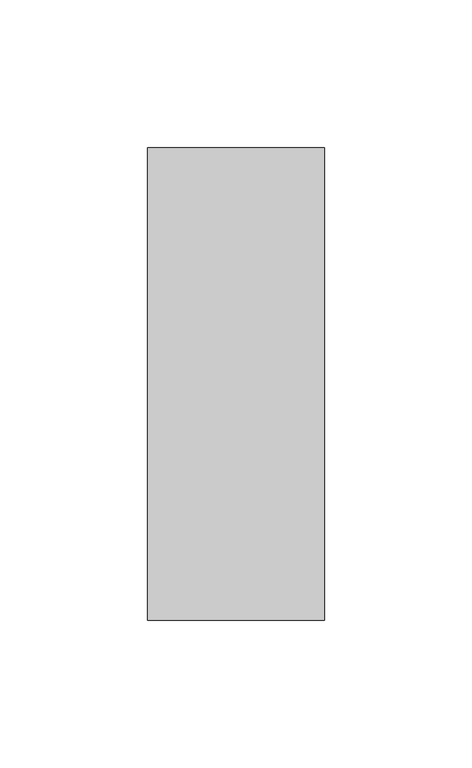
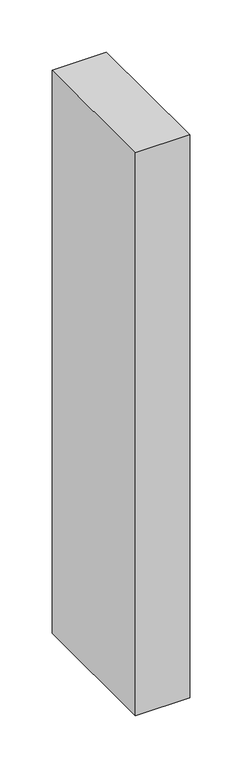
"""IFC4 building model written with IfcOpenShell, lengths in millimetres: column geometry, Madeira de lei-Coluna : Pontalete 6X16cm."""

import ifcopenshell
import ifcopenshell.guid

model = None  # the IFC model being written
_history = None  # IfcOwnerHistory: only IFC2X3 demands one
_inside = {}  # id of a spatial element -> (the spatial element, [elements in it])
_under = {}  # id of a project, library or spatial element -> (it, [spatial elements below it])
_declared = {}  # id of a project -> (the project, [libraries it declares])
_typed = {}  # id of a type object -> (the type object, [elements of that type])
_made_of = {}  # id of a material, layer set ... -> (it, [elements and type objects made of it])


def new_model(schema):
    """Start an empty IFC model of exactly this schema.

    Asked for "IFC4X3", IfcOpenShell would pick the latest addendum, in which some entities
    have other attributes; the version numbers below select the first issue.
    IFC2X3 requires an IfcOwnerHistory on every rooted entity: one is made here for all.
    """
    global model, _history
    if schema == "IFC4X3":
        model = ifcopenshell.file(schema_version=(4, 3, 0, 0))
    else:
        model = ifcopenshell.file(schema=schema)
    _inside.clear()
    _under.clear()
    _declared.clear()
    _typed.clear()
    _made_of.clear()
    _history = None
    if model.schema == "IFC2X3":
        org = make("IfcOrganization", Name="unknown")
        user = make(
            "IfcPersonAndOrganization",
            ThePerson=make("IfcPerson", FamilyName="unknown"),
            TheOrganization=org,
        )
        app = make(
            "IfcApplication",
            ApplicationDeveloper=org,
            Version="unknown",
            ApplicationFullName="unknown",
            ApplicationIdentifier="unknown",
        )
        _history = make(
            "IfcOwnerHistory",
            OwningUser=user,
            OwningApplication=app,
            ChangeAction="ADDED",
            CreationDate=0,
        )
    return model


def make(cls, **values):
    """One entity of the class cls with the attributes given. An attribute that is None is left unset."""
    return model.create_entity(
        cls, **{name: value for name, value in values.items() if value is not None}
    )


def rooted(cls, **values):
    """An entity with a GlobalId (a new one), such as an element, a storey or a relation."""
    return make(cls, GlobalId=ifcopenshell.guid.new(), OwnerHistory=_history, **values)


def si_unit(unit_type, name, prefix=None):
    """IfcSIUnit, for example si_unit("LENGTHUNIT", "METRE", prefix="MILLI")."""
    return make("IfcSIUnit", UnitType=unit_type, Prefix=prefix, Name=name)


def assignment(units):
    """IfcUnitAssignment: the units of a project."""
    return None if units is None else make("IfcUnitAssignment", Units=units)


def point(xyz):
    """IfcCartesianPoint."""
    return None if xyz is None else make("IfcCartesianPoint", Coordinates=xyz)


def direction(xyz):
    """IfcDirection."""
    return None if xyz is None else make("IfcDirection", DirectionRatios=xyz)


def frame(location, z_axis=None, x_axis=None):
    """IfcAxis2Placement3D, a coordinate frame: its origin and axes. An axis left out is left unset."""
    return make(
        "IfcAxis2Placement3D",
        Location=point(location),
        Axis=direction(z_axis),
        RefDirection=direction(x_axis),
    )


def origin():
    """The frame at (0, 0, 0) with its axes left unset."""
    return frame((0.0, 0.0, 0.0))


def place(relative_to, where):
    """IfcLocalPlacement: puts the frame where relative to a parent placement (None: the world)."""
    return make(
        "IfcLocalPlacement", PlacementRelTo=relative_to, RelativePlacement=where
    )


def context(
    kind, dimensions, precision=None, world=None, true_north=None, identifier=None
):
    """IfcGeometricRepresentationContext, for example the 3D "Model" context."""
    return make(
        "IfcGeometricRepresentationContext",
        ContextIdentifier=identifier,
        ContextType=kind,
        CoordinateSpaceDimension=dimensions,
        Precision=precision,
        WorldCoordinateSystem=world,
        TrueNorth=true_north,
    )


def project(units=None, contexts=None):
    """IfcProject with its units and contexts."""
    return rooted(
        "IfcProject",
        Name="project",
        RepresentationContexts=contexts,
        UnitsInContext=assignment(units),
    )


def spatial(cls, under=None, at=None, **own):
    """A site, building, storey or space (cls), placed at a placement, below another one or the project."""
    s = rooted(cls, ObjectPlacement=at, **own)
    if under is not None:
        _under.setdefault(under.id(), (under, []))[1].append(s)
    return s


def polyline(points):
    """IfcPolyline through the points."""
    return make("IfcPolyline", Points=[point(p) for p in points])


def outline(outer, holes=None, kind="AREA"):
    """IfcArbitraryClosedProfileDef: a profile drawn as a closed curve; with holes, ...WithVoids."""
    if holes is None:
        return make("IfcArbitraryClosedProfileDef", ProfileType=kind, OuterCurve=outer)
    return make(
        "IfcArbitraryProfileDefWithVoids",
        ProfileType=kind,
        OuterCurve=outer,
        InnerCurves=holes,
    )


def extrude(swept, where, along, depth):
    """IfcExtrudedAreaSolid: the profile swept, set in the frame where, extruded along a direction by depth."""
    return make(
        "IfcExtrudedAreaSolid",
        SweptArea=swept,
        Position=where,
        ExtrudedDirection=direction(along),
        Depth=depth,
    )


def shape(context_of_items, identifier, shape_type, items):
    """IfcShapeRepresentation: the items that make up one representation, for example the "Body"."""
    return make(
        "IfcShapeRepresentation",
        ContextOfItems=context_of_items,
        RepresentationIdentifier=identifier,
        RepresentationType=shape_type,
        Items=items,
    )


def source(mapping_origin, context_of_items, identifier, shape_type, items):
    """IfcRepresentationMap: a shape defined once, which mapped items show again and again."""
    return make(
        "IfcRepresentationMap",
        MappingOrigin=mapping_origin,
        MappedRepresentation=shape(context_of_items, identifier, shape_type, items),
    )


def transform(
    local_origin,
    x_axis=None,
    y_axis=None,
    z_axis=None,
    scale=None,
    scale2=None,
    scale3=None,
    uniform=True,
):
    """IfcCartesianTransformationOperator3D, or its non-uniform kind. x_axis, y_axis, z_axis: its Axis1, 2, 3."""
    if uniform:
        return make(
            "IfcCartesianTransformationOperator3D",
            Axis1=direction(x_axis),
            Axis2=direction(y_axis),
            LocalOrigin=point(local_origin),
            Scale=scale,
            Axis3=direction(z_axis),
        )
    return make(
        "IfcCartesianTransformationOperator3DnonUniform",
        Axis1=direction(x_axis),
        Axis2=direction(y_axis),
        LocalOrigin=point(local_origin),
        Scale=scale,
        Axis3=direction(z_axis),
        Scale2=scale2,
        Scale3=scale3,
    )


def mapped(mapping_source, mapping_target):
    """IfcMappedItem: shows the shape of a source again, moved by a transform."""
    return make(
        "IfcMappedItem", MappingSource=mapping_source, MappingTarget=mapping_target
    )


def made_of(thing, what):
    """Note that an element or type object is made of a material, layer set ...; save() writes the relation."""
    if what is not None:
        _made_of.setdefault(what.id(), (what, []))[1].append(thing)
    return thing


def element(
    cls,
    number,
    at=None,
    inside=None,
    cuts=None,
    type_object=None,
    material=None,
    context=None,
    identifier="Body",
    shape_type=None,
    held_by="IfcProductDefinitionShape",
    body=None,
    shapes=None,
    **own,
):
    """One element of the class cls, such as IfcWall. Its Tag is "e" and its number.

    at: its placement. inside: the storey or other place that contains it. cuts: it is an
    opening in that element (IfcRelVoidsElement). A single representation is given by context,
    identifier, shape_type and body (its items); several are given by shapes. held_by: the class
    of the entity that holds the representations. save() writes the other relations.
    """
    e = rooted(cls, Tag="e%d" % number, ObjectPlacement=at, **own)
    if body is not None:
        shapes = [shape(context, identifier, shape_type, body)]
    if shapes is not None:
        e.Representation = make(held_by, Representations=shapes)
    if inside is not None:
        _inside.setdefault(inside.id(), (inside, []))[1].append(e)
    if cuts is not None:
        rooted(
            "IfcRelVoidsElement", RelatingBuildingElement=cuts, RelatedOpeningElement=e
        )
    if type_object is not None:
        _typed.setdefault(type_object.id(), (type_object, []))[1].append(e)
    return made_of(e, material)


def aggregate(whole, parts):
    """IfcRelAggregates: a whole, such as a stair, and the parts it consists of."""
    return rooted("IfcRelAggregates", RelatingObject=whole, RelatedObjects=parts)


def save(model, path):
    """Write the relations noted so far, then the file.

    IfcRelAggregates (storeys below a building ...), IfcRelContainedInSpatialStructure (elements
    in a storey), IfcRelDefinesByType, IfcRelAssociatesMaterial and IfcRelDeclares: one each for
    every whole, place, type object, material and project.
    """
    for whole, parts in _under.values():
        aggregate(whole, parts)
    for where, things in _inside.values():
        rooted(
            "IfcRelContainedInSpatialStructure",
            RelatedElements=things,
            RelatingStructure=where,
        )
    for kind, things in _typed.values():
        rooted("IfcRelDefinesByType", RelatedObjects=things, RelatingType=kind)
    for what, things in _made_of.values():
        rooted("IfcRelAssociatesMaterial", RelatedObjects=things, RelatingMaterial=what)
    for by, libraries in _declared.values():
        rooted("IfcRelDeclares", RelatingContext=by, RelatedDefinitions=libraries)
    model.write(path)


def column_4db371bd(model_context):
    return source(origin(), model_context, "Body", "SweptSolid", [
        extrude(outline(polyline([(30.0, 80.0), (30.0, -80.0), (-30.0, -80.0), (-30.0, 80.0), (30.0, 80.0)])), frame((0.0, 0.0, 6710.0), z_axis=(0.0, 0.0, 1.0), x_axis=(1.0, 0.0, 0.0)), (0.0, 0.0, 1.0), 660.0),
    ])


if __name__ == "__main__":
    model = new_model("IFC4")
    model_context = context("Model", 3, world=origin())
    ifc_project = project(units=[si_unit("LENGTHUNIT", "METRE", prefix="MILLI")], contexts=[model_context])
    site = spatial("IfcSite", under=ifc_project)
    building = spatial("IfcBuilding", under=site)
    placement = place(None, origin())
    column_shape = column_4db371bd(model_context)
    element("IfcColumn", 1, ObjectType="Madeira de lei-Coluna : Pontalete 6X16cm", at=placement, inside=building, context=model_context, shape_type="MappedRepresentation", body=[
        mapped(column_shape, transform((0.0, 0.0, 0.0), x_axis=(1.0, 0.0, 0.0), y_axis=(0.0, 1.0, 0.0), z_axis=(0.0, 0.0, 1.0))),
    ])
    save(model, "model.ifc")

# Revit data of these elements
# Type "Madeira de lei-Coluna : Pontalete 6X16cm"
#   A = 0.01952 m²
#   b = 0.06 m
#   d = 0.16 m
#   Structural Material [instance default] = none
#   Assembly Code = ""
# Element 1 (IfcColumn, "Madeira de lei-Coluna : Pontalete 6X16cm")
#   Structural Material = .MADEIRAMENTO
#   Materials on its faces: ".MADEIRAMENTO"
# Materials
#   ".MADEIRAMENTO": class ".CC_MADEIRAS", colour RGB 212 179 113, transparency 0, Cost = 0
